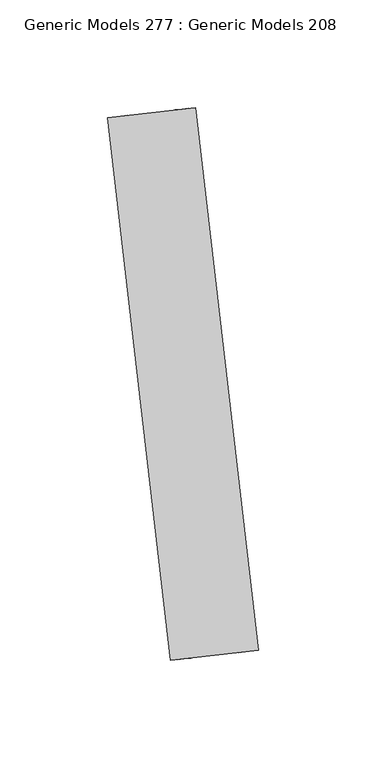
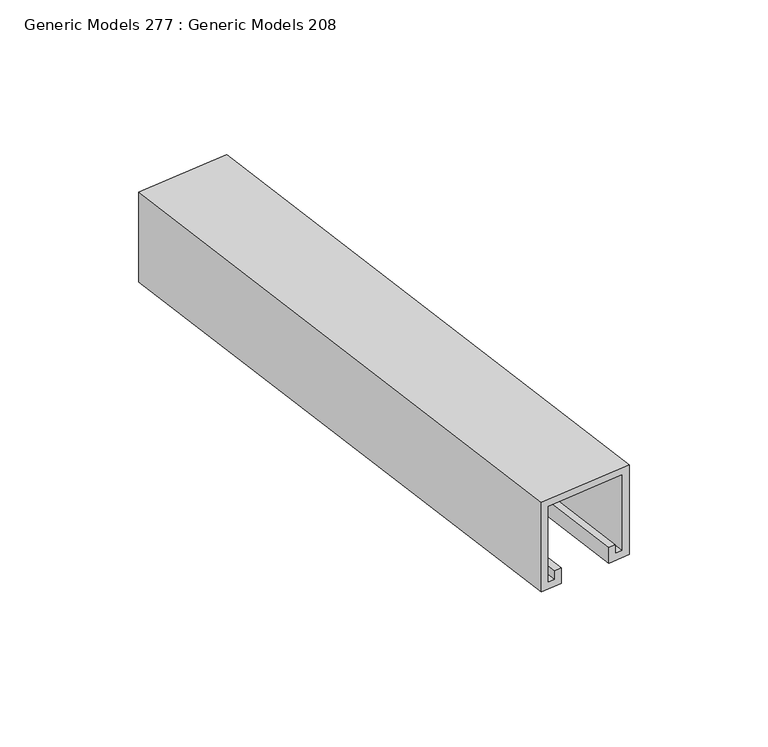
"""IFC4 building model written with IfcOpenShell, lengths in millimetres: proxy geometry, Generic Models 277 : Generic Models 208."""

from ifc_helpers import new_model, si_unit, frame, origin, place, context, project, spatial, polyline, outline, extrude, source, transform, mapped, element, save


def generic_models_277_generic_models_208_a1bbc452(model_context):
    return source(origin(), model_context, "Body", "SweptSolid", [
        extrude(outline(polyline([(-3.175, 0.0), (-3.175, 34.9249999), (-38.1, 34.9249999), (-38.1, 31.7499999), (-34.13125, 31.7499999), (-34.13125, 28.5749999), (-41.275, 28.5749999), (-41.275, 38.0999999), (0.0, 38.0999999), (0.0, -3.175), (-41.275, -3.175), (-41.275, 6.3499999), (-34.13125, 6.3499999), (-34.13125, 3.1749999), (-38.1, 3.1749999), (-38.1, 0.0), (-3.175, 0.0)])), frame((-1177.8886046, -22319.8306161, 1035.05), z_axis=(-0.11558924632698354, 0.9932970986233475, 0.0), x_axis=(0.0, 0.0, 1.0)), (0.0, 0.0, 1.0), 254.0),
    ])


if __name__ == "__main__":
    model = new_model("IFC4")
    model_context = context("Model", 3, world=origin())
    ifc_project = project(units=[si_unit("LENGTHUNIT", "METRE", prefix="MILLI")], contexts=[model_context])
    site = spatial("IfcSite", under=ifc_project)
    building = spatial("IfcBuilding", under=site)
    placement = place(None, origin())
    generic_models_277_generic_models_208_shape = generic_models_277_generic_models_208_a1bbc452(model_context)
    element("IfcBuildingElementProxy", 1, Name="Generic Models 277 : Generic Models 208", ObjectType="Generic Models 277 : Generic Models 208", at=placement, inside=building, context=model_context, shape_type="MappedRepresentation", body=[
        mapped(generic_models_277_generic_models_208_shape, transform((0.0, 0.0, 0.0), x_axis=(1.0, 0.0, 0.0), y_axis=(0.0, 1.0, 0.0), z_axis=(0.0, 0.0, 1.0))),
    ])
    save(model, "model.ifc")

# Revit data of these elements
# Element 1 (IfcBuildingElementProxy, "Generic Models 277 : Generic Models 208")
#   Materials on its faces: "UNISTRUT P1000, 1 5/8\" X 1 5/8\", CHANNEL OR ALUM. CHANNEL"
# Materials
#   "UNISTRUT P1000, 1 5/8\" X 1 5/8\", CHANNEL OR ALUM. CHANNEL": class "Metal", colour RGB 244 244 244, transparency 0, Description = "Aluminum 6061", Cost = 0
